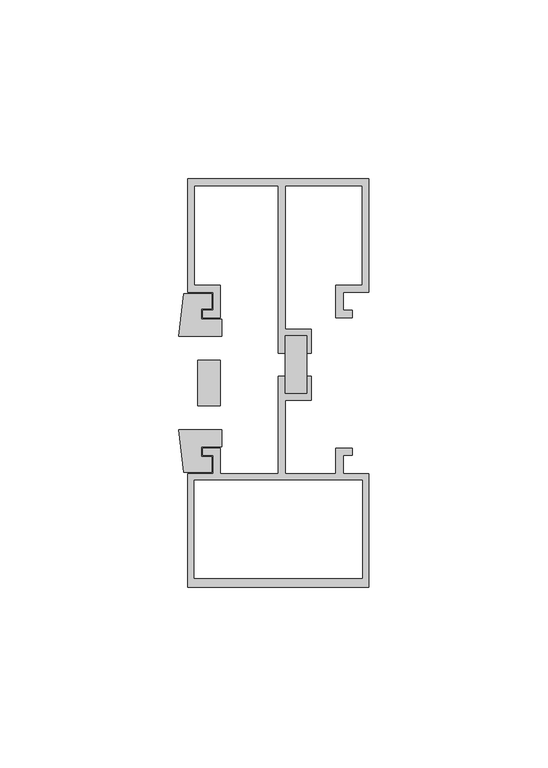
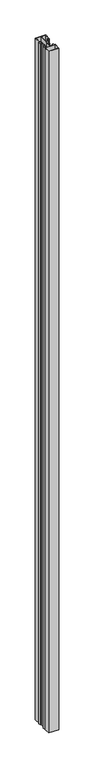
"""IFC4 building model written with IfcOpenShell, lengths in millimetres: proxy geometry, Generic Models 3:Generic Models 1:5:Generic Models 1:5 : Generic Models 3:Generic Models 1:300625:345888:Generic Models 1:5:Generic Models 1:5 : Generic Models 3:Generic Models 1:300625:345888 : Generic Models 3:Generic Models 1:5:Generic Models 1:5 : Generic Models 3:Generic Models 1:300625:345888:2 : Generic Models 3:Generic Models 1:5:Generic Models 1:5 : Generic Models 3:Generic Models 1:300625:345888:Generic Models 1:5:Generic Models 1:5 : Generic Models 3:Generic Models 1:300625:345888 : Generic Models 3:Generic Models 1:5:Generic Models 1:5 : Generic Models 3:Generic Models 1:300625:345888:301574."""

from ifc_helpers import new_model, si_unit, frame, origin, place, context, project, spatial, polyline, outline, extrude, source, transform, mapped, element, save


def generic_models_c8556d47(model_context):
    return source(origin(), model_context, "Body", "SweptSolid", [
        extrude(outline(polyline([(593708.2535457, -579063.9802804), (593708.2535457, -579047.8688442), (593714.333333, -579047.8688442), (593714.333333, -579063.9802804), (593708.2535457, -579063.9802804)])), frame((0.0, 0.0, 66.3122056), z_axis=(0.0, 0.0, 1.0), x_axis=(1.0, 0.0, 0.0)), (0.0, 0.0, 1.0), 3584.971571),
        extrude(outline(polyline([(593683.8226303, -579067.3663841), (593683.8226303, -579054.6663841), (593690.1661787, -579054.6663841), (593690.1661787, -579067.3663841), (593683.8226303, -579067.3663841)])), frame((0.0, 0.0, 66.3122056), z_axis=(0.0, 0.0, 1.0), x_axis=(1.0, 0.0, 0.0)), (0.0, 0.0, 1.0), 3584.971571),
        extrude(outline(polyline([(593684.8495131, -579078.8588708), (593684.8495131, -579081.704549), (593687.7933729, -579081.704549), (593687.7933729, -579086.0026208), (593679.9536635, -579086.0026208), (593678.4927966, -579074.1048149), (593690.5630537, -579074.1048149), (593690.5630537, -579078.8588708), (593684.8495131, -579078.8588708)])), frame((0.0, 0.0, 66.3122056), z_axis=(0.0, 0.0, 1.0), x_axis=(1.0, 0.0, 0.0)), (0.0, 0.0, 1.0), 3584.971571),
        extrude(outline(polyline([(593679.9536635, -579036.0301474), (593687.7933729, -579036.0301474), (593687.7933729, -579040.3282192), (593684.8495131, -579040.3282192), (593684.8495131, -579043.1738974), (593690.5630537, -579043.1738974), (593690.5630537, -579047.9279532), (593678.4927966, -579047.9279532), (593679.9536635, -579036.0301474)])), frame((0.0, 0.0, 66.3122056), z_axis=(0.0, 0.0, 1.0), x_axis=(1.0, 0.0, 0.0)), (0.0, 0.0, 1.0), 3584.9377944),
        extrude(outline(polyline([(593731.7367239, -579118.1663841), (593680.9705005, -579118.1663841), (593680.9705005, -579086.3994958), (593688.1902479, -579086.3994958), (593688.1902479, -579081.307674), (593685.2463881, -579081.307674), (593685.2463881, -579079.2557458), (593690.1661787, -579079.2557458), (593690.1661787, -579086.3994958), (593706.3536122, -579086.3994958), (593706.3536122, -579059.1164506), (593708.2535457, -579059.1164506), (593708.2535457, -579063.9802804), (593714.333333, -579063.9802804), (593714.333333, -579059.1164506), (593715.6252878, -579059.1164506), (593715.6252878, -579065.8802139), (593708.2535457, -579065.8802139), (593708.2535457, -579086.3994958), (593722.4650484, -579086.3994958), (593722.4650484, -579079.2557458), (593727.036208, -579079.2557458), (593727.036208, -579081.307674), (593724.5169766, -579081.307674), (593724.5169766, -579086.3994958), (593731.7367239, -579086.3994958), (593731.7367239, -579118.1663841)]), holes=[polyline([(593682.870434, -579088.2994293), (593682.870434, -579115.6584719), (593729.8367904, -579115.6584719), (593729.8367904, -579088.2994293), (593682.870434, -579088.2994293)])]), frame((0.0, 0.0, 66.3122056), z_axis=(0.0, 0.0, 1.0), x_axis=(1.0, 0.0, 0.0)), (0.0, 0.0, 1.0), 3584.971571),
        extrude(outline(polyline([(593685.2463881, -579040.7250942), (593688.1902479, -579040.7250942), (593688.1902479, -579035.6332724), (593680.9705005, -579035.6332724), (593680.9705005, -579003.8663841), (593731.7367239, -579003.8663841), (593731.7367239, -579035.6332724), (593724.5169766, -579035.6332724), (593724.5169766, -579040.7250942), (593727.036208, -579040.7250942), (593727.036208, -579042.7770224), (593722.4650484, -579042.7770224), (593722.4650484, -579033.7333389), (593729.8145113, -579033.7333389), (593729.8145113, -579005.8423149), (593708.2535457, -579005.8423149), (593708.2535457, -579045.9689107), (593715.6252878, -579045.9689107), (593715.6252878, -579052.732674), (593714.333333, -579052.732674), (593714.333333, -579047.8688442), (593708.2535457, -579047.8688442), (593708.2535457, -579052.732674), (593706.3536122, -579052.732674), (593706.3536122, -579005.8423149), (593682.8802996, -579005.8423149), (593682.8802996, -579033.7333389), (593690.1661787, -579033.7333389), (593690.1661787, -579042.7770224), (593685.2463881, -579042.7770224), (593685.2463881, -579040.7250942)])), frame((0.0, 0.0, 66.3122056), z_axis=(0.0, 0.0, 1.0), x_axis=(1.0, 0.0, 0.0)), (0.0, 0.0, 1.0), 3584.971571),
    ])


if __name__ == "__main__":
    model = new_model("IFC4")
    model_context = context("Model", 3, world=origin())
    ifc_project = project(units=[si_unit("LENGTHUNIT", "METRE", prefix="MILLI")], contexts=[model_context])
    site = spatial("IfcSite", under=ifc_project)
    building = spatial("IfcBuilding", under=site)
    placement = place(None, origin())
    generic_models_shape = generic_models_c8556d47(model_context)
    element("IfcBuildingElementProxy", 1, Name="Generic Models 3:Generic Models 1:5:Generic Models 1:5 : Generic Models 3:Generic Models 1:300625:345888:Generic Models 1:5:Generic Models 1:5 : Generic Models 3:Generic Models 1:300625:345888 : Generic Models 3:Generic Models 1:5:Generic Models 1:5 : Generic Models 3:Generic Models 1:300625:345888:2 : Generic Models 3:Generic Models 1:5:Generic Models 1:5 : Generic Models 3:Generic Models 1:300625:345888:Generic Models 1:5:Generic Models 1:5 : Generic Models 3:Generic Models 1:300625:345888 : Generic Models 3:Generic Models 1:5:Generic Models 1:5 : Generic Models 3:Generic Models 1:300625:345888:301574", ObjectType="Generic Models 3:Generic Models 1:5:Generic Models 1:5 : Generic Models 3:Generic Models 1:300625:345888:Generic Models 1:5:Generic Models 1:5 : Generic Models 3:Generic Models 1:300625:345888 : Generic Models 3:Generic Models 1:5:Generic Models 1:5 : Generic Models 3:Generic Models 1:300625:345888:2 : Generic Models 3:Generic Models 1:5:Generic Models 1:5 : Generic Models 3:Generic Models 1:300625:345888:Generic Models 1:5:Generic Models 1:5 : Generic Models 3:Generic Models 1:300625:345888 : Generic Models 3:Generic Models 1:5:Generic Models 1:5 : Generic Models 3:Generic Models 1:300625:345888:301574", at=placement, inside=building, context=model_context, shape_type="MappedRepresentation", body=[
        mapped(generic_models_shape, transform((0.0, 0.0, 0.0), x_axis=(1.0, 0.0, 0.0), y_axis=(0.0, 1.0, 0.0), z_axis=(0.0, 0.0, 1.0))),
    ])
    save(model, "model.ifc")

# Revit data of these elements
# Type "Generic Models 3:Generic Models 1:5:Generic Models 1:5 : Generic Models 3:Generic Models 1:300625:345888:Generic Models 1:5:Generic Models 1:5 : Generic Models 3:Generic Models 1:300625:345888 : Generic Models 3:Generic Models 1:5:Generic Models 1:5 : Generic Models 3:Generic Models 1:300625:345888:2 : Generic Models 3:Generic Models 1:5:Generic Models 1:5 : Generic Models 3:Generic Models 1:300625:345888:Generic Models 1:5:Generic Models 1:5 : Generic Models 3:Generic Models 1:300625:345888 : Generic Models 3:Generic Models 1:5:Generic Models 1:5 : Generic Models 3:Generic Models 1:300625:345888:301574"
#   NameOverride = "Generic Models 3:Generic Models 1:5:Generic Models 1:5 : Generic Models 3:Generic Models 1:300625:345888:Generic Models 1:5:Generic Models 1:5 : Generic Models 3:Generic Models 1:300625:345888 : Generic Models 3:Generic Models 1:5:Generic Models 1:5 : Generic Models 3:Generic Models 1:300625:345888:301574"
#   ObjectTypeOverride = "Generic Models 1:5:Generic Models 1:5 : Generic Models 3:Generic Models 1:300625:345888 : Generic Models 3:Generic Models 1:5:Generic Models 1:5 : Generic Models 3:Generic Models 1:300625:345888"
#   Reference = "Generic Models 1"
#   Tag = "301574"
# Element 1 (IfcBuildingElementProxy, "Generic Models 3:Generic Models 1:5:Generic Models 1:5 : Generic Models 3:Generic Models 1:300625:345888:Generic Models 1:5:Generic Models 1:5 : Generic Models 3:Generic Models 1:300625:345888 : Generic Models 3:Generic Models 1:5:Generic Models 1:5 : Generic Models 3:Generic Models 1:300625:345888:2 : Generic Models 3:Generic Models 1:5:Generic Models 1:5 : Generic Models 3:Generic Models 1:300625:345888:Generic Models 1:5:Generic Models 1:5 : Generic Models 3:Generic Models 1:300625:345888 : Generic Models 3:Generic Models 1:5:Generic Models 1:5 : Generic Models 3:Generic Models 1:300625:345888:301574")
#   Materials on its faces: "THERMAL BROKEN ALUMINUM STOREFRONT", "Compression Gasket_1", "Desiccant Sealant_1"
# Materials
#   "THERMAL BROKEN ALUMINUM STOREFRONT": class "Unassigned", colour RGB 244 244 244, transparency 0, Cost = 0
#   "Compression Gasket_1": class "Unassigned", colour RGB 178 178 178, transparency 0
#   "Desiccant Sealant_1": class "Unassigned", colour RGB 120 120 120, transparency 0
